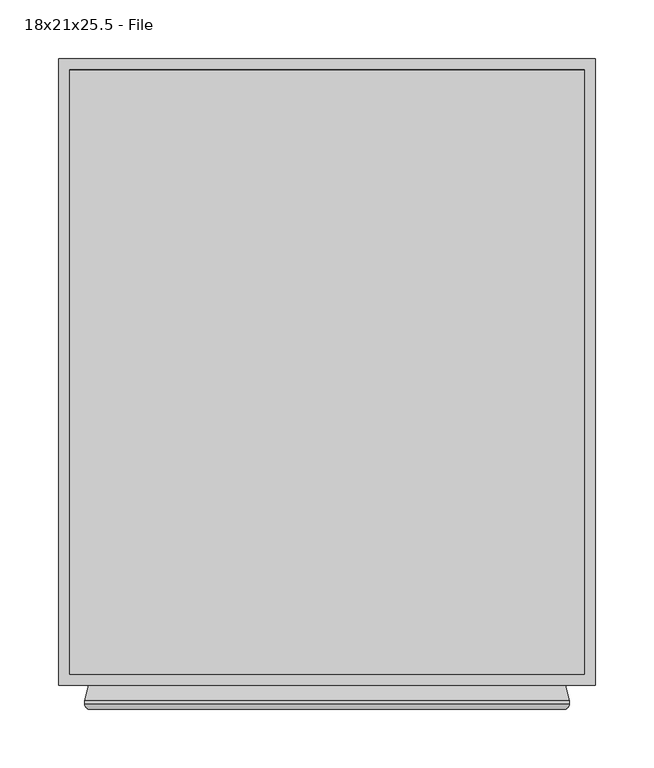
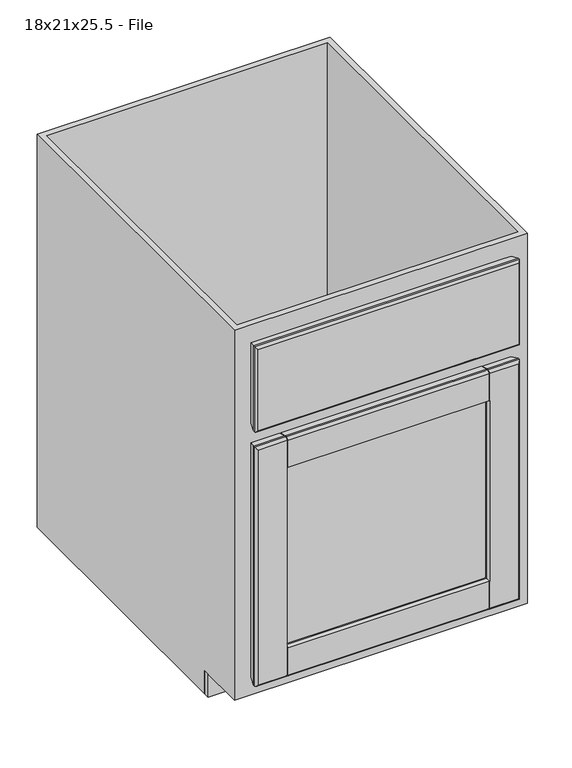
"""IFC4 building model written with IfcOpenShell, lengths in millimetres: furniture geometry, Cabinet-Base-Merillat-Single_Door-Marlin : 18x21x25.5 - File."""

from ifc_helpers import new_model, si_unit, frame, origin, origin_with_axes, place, context, project, spatial, polyline, circle_curve, ellipse_curve, outline, extrude, faceted_brep, source, transform, mapped, element, save
from ifc_brep_helpers import plane_surface, cylinder_surface, advanced_brep


def furniture_18x21x25_5_file_292c1ec0(model_context):
    return source(origin(), model_context, "Body", "SolidModel", [
        advanced_brep(
        [(225.1127049, -625.4496, 457.2), (222.0162124, -629.92, 454.1035075), (222.0162124, -629.92, 66.5964925), (225.1127049, -625.4496, 63.5), (225.1127049, -622.681, 63.5), (225.1127049, -622.681, 457.2), (221.6075049, -609.6, 67.0052), (221.6075049, -609.6, 453.6948), (176.9115422, -609.6, 408.9988372), (176.9115422, -609.6, 111.7011628), (176.5414105, -610.39375, 112.0712945), (174.4602514, -614.85681, 114.1524535), (174.4602514, -614.85681, 406.5475465), (176.5414105, -610.39375, 408.6287055), (175.8600209, -617.0969093, 112.752684), (175.8600209, -617.0969093, 407.947316), (190.1877049, -617.347, 98.425), (190.1877049, -617.347, 422.275), (190.1877049, -622.173, 98.425), (190.1877049, -622.173, 422.275), (175.8600209, -622.4230907, 112.752684), (175.8600209, -622.4230907, 407.947316), (174.4602514, -624.66319, 114.1524535), (174.4602514, -624.66319, 406.5475465), (176.5414105, -629.12625, 112.0712945), (176.9086747, -629.9138508, 111.7040302), (176.9115422, -629.92, 408.9988372), (176.5414105, -629.12625, 408.6287055), (176.9086747, -629.92, 66.5964925), (176.9086747, -625.4496, 63.5), (-184.5408026, -629.92, 66.5964925), (-187.6372951, -625.4496, 63.5), (-139.4730764, -625.4496, 63.5), (-139.4730764, -629.92, 66.5964925), (175.3211747, -625.4496, 63.5), (175.3211747, -629.92, 66.5964925), (-137.8855764, -629.92, 66.5964925), (-137.8855764, -625.4496, 63.5), (176.9086747, -622.681, 63.5), (-187.6372951, -622.681, 63.5), (-139.4730764, -622.681, 63.5), (175.3211747, -622.681, 63.5), (-137.8855764, -622.681, 63.5), (176.9086747, -609.6, 67.0052), (-184.1320951, -609.6, 67.0052), (-139.4730764, -609.6, 67.0052), (175.3211747, -609.6, 67.0052), (-137.8855764, -609.6, 67.0052), (-136.9848416, -614.85681, 114.1524535), (175.3211747, -610.39375, 112.0712945), (175.3211747, -609.6, 111.7011628), (-137.8855764, -609.6, 111.7011628), (-137.8855764, -610.39375, 112.0712945), (-139.0660006, -610.39375, 112.0712945), (-138.384611, -617.0969093, 112.752684), (-152.7122951, -617.347, 98.425), (-152.7122951, -622.173, 98.425), (-138.384611, -622.4230907, 112.752684), (-136.9848416, -624.66319, 114.1524535), (-139.0660006, -629.12625, 112.0712945), (-137.8855764, -629.12625, 112.0712945), (-137.8855764, -629.92, 111.7011628), (175.3211747, -629.92, 111.7011628), (175.3211747, -629.12625, 112.0712945), (-184.5408026, -629.92, 454.1035075), (-187.6372951, -625.4496, 457.2), (-187.6372951, -622.681, 457.2), (-184.1320951, -609.6, 453.6948), (-139.4361323, -609.6, 111.7011628), (-139.4361323, -609.6, 408.9988372), (-139.0660006, -610.39375, 408.6287055), (-136.9848416, -614.85681, 406.5475465), (-138.384611, -617.0969093, 407.947316), (-152.7122951, -617.347, 422.275), (-152.7122951, -622.173, 422.275), (-138.384611, -622.4230907, 407.947316), (-136.9848416, -624.66319, 406.5475465), (-139.0660006, -629.12625, 408.6287055), (-139.4361323, -629.92, 408.9988372), (-139.4361323, -629.92, 111.7011628), (-139.4730764, -629.92, 454.1035075), (-139.4730764, -625.4496, 457.2), (176.9086747, -625.4496, 457.2), (176.9086747, -629.92, 454.1035075), (-137.8855764, -625.4496, 457.2), (-137.8855764, -629.92, 454.1035075), (175.3211747, -629.92, 454.1035075), (175.3211747, -625.4496, 457.2), (-139.4730764, -622.681, 457.2), (176.9086747, -622.681, 457.2), (-137.8855764, -622.681, 457.2), (175.3211747, -622.681, 457.2), (-139.4730764, -609.6, 453.6948), (176.9086747, -609.6, 453.6948), (-137.8855764, -609.6, 453.6948), (175.3211747, -609.6, 453.6948), (-137.8855764, -609.6, 408.9988372), (175.3211747, -609.6, 408.9988372), (-137.8855764, -610.39375, 408.6287055), (175.3211747, -610.39375, 408.6287055), (175.3211747, -629.12625, 408.6287055), (175.3211747, -629.92, 408.9988372), (-137.8855764, -629.92, 408.9988372), (-137.8855764, -629.12625, 408.6287055), (-137.8855764, -610.39375, 453.0857412), (-137.8855764, -622.7855037, 456.40625), (-137.8855764, -625.4496, 456.40625), (-137.8855764, -629.12625, 453.9526052), (-139.4730764, -629.12625, 408.6287055), (-139.4730764, -629.12625, 453.9526052), (-139.4730764, -625.4496, 456.40625), (-139.4730764, -622.7855037, 456.40625), (-139.4730764, -610.39375, 453.0857412), (-139.4730764, -610.39375, 408.6287055), (176.9086747, -610.39375, 408.6287055), (176.9086747, -610.39375, 453.0857412), (176.9086747, -622.7855037, 456.40625), (176.9086747, -625.4496, 456.40625), (176.9086747, -629.12625, 453.9526052), (176.9086747, -629.12625, 408.6287055), (175.3211747, -629.12625, 453.9526052), (175.3211747, -625.4496, 456.40625), (175.3211747, -622.7855037, 456.40625), (175.3211747, -610.39375, 453.0857412), (176.9086747, -629.12625, 112.0712945), (176.9086747, -629.12625, 66.7473948), (176.9086747, -625.4496, 64.29375), (176.9086747, -622.7855037, 64.29375), (176.9086747, -610.39375, 67.6142588), (176.9086747, -610.39375, 112.0712945), (175.3211747, -610.39375, 67.6142588), (175.3211747, -622.7855037, 64.29375), (175.3211747, -625.4496, 64.29375), (175.3211747, -629.12625, 66.7473948), (-137.8855764, -629.12625, 66.7473948), (-137.8855764, -625.4496, 64.29375), (-137.8855764, -622.7855037, 64.29375), (-137.8855764, -610.39375, 67.6142588), (-139.4730764, -629.12625, 112.0712945), (-139.4730764, -610.39375, 112.0712945), (-139.4730764, -610.39375, 67.6142588), (-139.4730764, -622.7855037, 64.29375), (-139.4730764, -625.4496, 64.29375), (-139.4730764, -629.12625, 66.7473948)],
        [
            (0, 1, ellipse_curve(frame((220.3375049, -625.4496, 452.4248), z_axis=(0.7071067811865475, 0.0, -0.7071067811865475), x_axis=(0.7071067811865474, 0.0, 0.7071067811865476)), 6.7531526, 4.7752)),
            (1, 2),
            (2, 3, ellipse_curve(frame((220.3375049, -625.4496, 68.2752), z_axis=(0.7071067811865475, 0.0, 0.7071067811865475), x_axis=(-0.7071067811865474, 0.0, 0.7071067811865476)), 6.7531526, 4.7752)),
            (3, 0),
            (3, 4),
            (4, 5),
            (5, 0),
            (4, 6),
            (6, 7),
            (7, 5),
            (8, 9),
            (9, 10),
            (10, 11),
            (11, 12),
            (12, 13),
            (13, 8),
            (11, 14, ellipse_curve(frame((175.8875049, -615.5223492, 112.7252), z_axis=(0.7071067811865475, 0.0, 0.7071067811865475), x_axis=(-0.7071067811865474, 0.0, 0.7071067811865476)), 2.2271035, 1.5748)),
            (14, 15),
            (15, 12, ellipse_curve(frame((175.8875049, -615.5223492, 407.9748), z_axis=(0.7071067811865475, 0.0, -0.7071067811865475), x_axis=(0.7071067811865474, 0.0, 0.7071067811865476)), 2.2271035, 1.5748)),
            (14, 16),
            (16, 17),
            (17, 15),
            (16, 18),
            (18, 19),
            (19, 17),
            (18, 20),
            (20, 21),
            (21, 19),
            (20, 22, ellipse_curve(frame((175.8875049, -623.9976508, 112.7252), z_axis=(0.7071067811865475, 0.0, 0.7071067811865475), x_axis=(-0.7071067811865474, 0.0, 0.7071067811865476)), 2.2271035, 1.5748)),
            (22, 23),
            (23, 21, ellipse_curve(frame((175.8875049, -623.9976508, 407.9748), z_axis=(0.7071067811865475, 0.0, -0.7071067811865475), x_axis=(0.7071067811865474, 0.0, 0.7071067811865476)), 2.2271035, 1.5748)),
            (22, 24),
            (24, 25),
            (25, 26),
            (26, 27),
            (27, 23),
            (2, 28),
            (28, 29, circle_curve(frame((176.9086747, -625.4496, 68.2752), z_axis=(1.0, 0.0, 0.0), x_axis=(0.0, 1.0, 0.0)), 4.7752)),
            (29, 3),
            (30, 31, ellipse_curve(frame((-182.8620951, -625.4496, 68.2752), z_axis=(0.7071067811865475, 0.0, -0.7071067811865475), x_axis=(0.7071067811865476, 0.0, 0.7071067811865474)), 6.7531526, 4.7752)),
            (31, 32),
            (32, 33, circle_curve(frame((-139.4730764, -625.4496, 68.2752), z_axis=(-1.0, 0.0, 0.0), x_axis=(0.0, 1.0, 0.0)), 4.7752)),
            (33, 30),
            (34, 35, circle_curve(frame((175.3211747, -625.4496, 68.2752), z_axis=(-1.0, 0.0, 0.0), x_axis=(0.0, 1.0, 0.0)), 4.7752)),
            (35, 36),
            (36, 37, circle_curve(frame((-137.8855764, -625.4496, 68.2752), z_axis=(1.0, 0.0, 0.0), x_axis=(0.0, 1.0, 0.0)), 4.7752)),
            (37, 34),
            (29, 38),
            (38, 4),
            (31, 39),
            (39, 40),
            (40, 32),
            (41, 34),
            (37, 42),
            (42, 41),
            (38, 43),
            (43, 6),
            (39, 44),
            (44, 45),
            (45, 40),
            (46, 41),
            (42, 47),
            (47, 46),
            (48, 11),
            (10, 49),
            (49, 50),
            (50, 51),
            (51, 52),
            (52, 53),
            (53, 48),
            (48, 54, ellipse_curve(frame((-138.4120951, -615.5223492, 112.7252), z_axis=(0.7071067811865475, 0.0, -0.7071067811865475), x_axis=(0.7071067811865476, 0.0, 0.7071067811865474)), 2.2271035, 1.5748)),
            (54, 14),
            (54, 55),
            (55, 16),
            (55, 56),
            (56, 18),
            (56, 57),
            (57, 20),
            (57, 58, ellipse_curve(frame((-138.4120951, -623.9976508, 112.7252), z_axis=(0.7071067811865475, 0.0, -0.7071067811865475), x_axis=(0.7071067811865476, 0.0, 0.7071067811865474)), 2.2271035, 1.5748)),
            (58, 22),
            (58, 59),
            (59, 60),
            (60, 61),
            (61, 62),
            (62, 63),
            (63, 24),
            (30, 64),
            (64, 65, ellipse_curve(frame((-182.8620951, -625.4496, 452.4248), z_axis=(-0.7071067811865475, 0.0, -0.7071067811865475), x_axis=(0.7071067811865474, 0.0, -0.7071067811865476)), 6.7531526, 4.7752)),
            (65, 31),
            (65, 66),
            (66, 39),
            (66, 67),
            (67, 44),
            (68, 69),
            (69, 70),
            (70, 71),
            (71, 48),
            (53, 68),
            (71, 72, ellipse_curve(frame((-138.4120951, -615.5223492, 407.9748), z_axis=(-0.7071067811865475, 0.0, -0.7071067811865475), x_axis=(0.7071067811865474, 0.0, -0.7071067811865476)), 2.2271035, 1.5748)),
            (72, 54),
            (72, 73),
            (73, 55),
            (73, 74),
            (74, 56),
            (74, 75),
            (75, 57),
            (75, 76, ellipse_curve(frame((-138.4120951, -623.9976508, 407.9748), z_axis=(-0.7071067811865475, 0.0, -0.7071067811865475), x_axis=(0.7071067811865474, 0.0, -0.7071067811865476)), 2.2271035, 1.5748)),
            (76, 58),
            (76, 77),
            (77, 78),
            (78, 79),
            (79, 59),
            (64, 80),
            (80, 81, circle_curve(frame((-139.4730764, -625.4496, 452.4248), z_axis=(-1.0, 0.0, 0.0), x_axis=(0.0, 1.0, 0.0)), 4.7752)),
            (81, 65),
            (0, 82),
            (82, 83, circle_curve(frame((176.9086747, -625.4496, 452.4248), z_axis=(1.0, 0.0, 0.0), x_axis=(0.0, 1.0, 0.0)), 4.7752)),
            (83, 1),
            (84, 85, circle_curve(frame((-137.8855764, -625.4496, 452.4248), z_axis=(1.0, 0.0, 0.0), x_axis=(0.0, 1.0, 0.0)), 4.7752)),
            (85, 86),
            (86, 87, circle_curve(frame((175.3211747, -625.4496, 452.4248), z_axis=(-1.0, 0.0, 0.0), x_axis=(0.0, 1.0, 0.0)), 4.7752)),
            (87, 84),
            (81, 88),
            (88, 66),
            (5, 89),
            (89, 82),
            (90, 84),
            (87, 91),
            (91, 90),
            (88, 92),
            (92, 67),
            (7, 93),
            (93, 89),
            (94, 90),
            (91, 95),
            (95, 94),
            (43, 9),
            (8, 93),
            (92, 69),
            (68, 45),
            (96, 94),
            (95, 97),
            (97, 96),
            (50, 46),
            (47, 51),
            (12, 71),
            (70, 98),
            (98, 96),
            (97, 99),
            (99, 13),
            (15, 72),
            (17, 73),
            (19, 74),
            (21, 75),
            (23, 76),
            (27, 100),
            (100, 101),
            (101, 102),
            (102, 103),
            (103, 77),
            (83, 26),
            (25, 28),
            (33, 79),
            (78, 80),
            (85, 102),
            (101, 86),
            (35, 62),
            (61, 36),
            (98, 104),
            (104, 105),
            (105, 106),
            (106, 107, circle_curve(frame((-137.8855764, -625.4496, 452.4248), z_axis=(1.0, 0.0, 0.0), x_axis=(0.0, 0.0, 1.0)), 3.98145)),
            (107, 103),
            (78, 108),
            (108, 109),
            (109, 110, circle_curve(frame((-139.4730764, -625.4496, 452.4248), z_axis=(-1.0, 0.0, 0.0), x_axis=(0.0, 0.0, 1.0)), 3.98145)),
            (110, 111),
            (111, 112),
            (112, 113),
            (113, 69),
            (77, 108),
            (107, 109),
            (106, 110),
            (105, 111),
            (104, 112),
            (70, 113),
            (8, 114),
            (114, 115),
            (115, 116),
            (116, 117),
            (117, 118, circle_curve(frame((176.9086747, -625.4496, 452.4248), z_axis=(1.0, 0.0, 0.0), x_axis=(0.0, 0.0, 1.0)), 3.98145)),
            (118, 119),
            (119, 26),
            (100, 120),
            (120, 121, circle_curve(frame((175.3211747, -625.4496, 452.4248), z_axis=(-1.0, 0.0, 0.0), x_axis=(0.0, 0.0, 1.0)), 3.98145)),
            (121, 122),
            (122, 123),
            (123, 99),
            (119, 27),
            (118, 120),
            (117, 121),
            (116, 122),
            (115, 123),
            (114, 13),
            (25, 124),
            (124, 125),
            (125, 126, circle_curve(frame((176.9086747, -625.4496, 68.2752), z_axis=(1.0, 0.0, 0.0), x_axis=(0.0, 0.0, 1.0)), 3.98145)),
            (126, 127),
            (127, 128),
            (128, 129),
            (129, 9),
            (49, 130),
            (130, 131),
            (131, 132),
            (132, 133, circle_curve(frame((175.3211747, -625.4496, 68.2752), z_axis=(-1.0, 0.0, 0.0), x_axis=(0.0, 0.0, 1.0)), 3.98145)),
            (133, 63),
            (129, 10),
            (128, 130),
            (127, 131),
            (126, 132),
            (125, 133),
            (124, 24),
            (60, 134),
            (134, 135, circle_curve(frame((-137.8855764, -625.4496, 68.2752), z_axis=(1.0, 0.0, 0.0), x_axis=(0.0, 0.0, 1.0)), 3.98145)),
            (135, 136),
            (136, 137),
            (137, 52),
            (138, 79),
            (68, 139),
            (139, 140),
            (140, 141),
            (141, 142),
            (142, 143, circle_curve(frame((-139.4730764, -625.4496, 68.2752), z_axis=(-1.0, 0.0, 0.0), x_axis=(0.0, 0.0, 1.0)), 3.98145)),
            (143, 138),
            (138, 59),
            (53, 139),
            (137, 140),
            (136, 141),
            (135, 142),
            (134, 143),
        ],
        [
            cylinder_surface(frame((220.3375049, -625.4496, 457.2), z_axis=(0.0, 0.0, 1.0), x_axis=(0.0, 1.0, 0.0)), 4.7752),
            plane_surface(frame((225.1127049, -625.4496, 457.2), z_axis=(1.0, 0.0, 0.0), x_axis=(0.0, 0.0, -1.0))),
            plane_surface(frame((225.1127049, -622.681, 457.2), z_axis=(0.9659229350723619, 0.25882983502910506, 0.0), x_axis=(0.0, 0.0, -1.0))),
            plane_surface(frame((176.9115422, -609.6, 408.9988372), z_axis=(-0.9063077870366099, 0.4226182617407856, 0.0), x_axis=(0.0, 0.0, -1.0))),
            cylinder_surface(frame((175.8875049, -615.5223492, 457.2), z_axis=(0.0, 0.0, 1.0000000000000002), x_axis=(-0.01745240643729364, -0.9998476951563912, 0.0)), 1.5748),
            plane_surface(frame((175.8600209, -617.0969093, 407.947316), z_axis=(-0.017452406437322144, -0.9998476951563906, 0.0), x_axis=(0.0, 0.0, -1.0))),
            plane_surface(frame((190.1877049, -617.347, 422.275), z_axis=(-1.0, 0.0, 0.0), x_axis=(0.0, 0.0, -1.0))),
            plane_surface(frame((190.1877049, -622.173, 422.275), z_axis=(-0.01745240643727848, 0.9998476951563914, 0.0), x_axis=(0.0, 0.0, -1.0))),
            cylinder_surface(frame((175.8875049, -623.9976508, 457.2), z_axis=(0.0, 0.0, 1.0000000000000002), x_axis=(-0.9063077870367326, -0.42261826174052236, 0.0)), 1.5748),
            plane_surface(frame((174.4602514, -624.66319, 406.5475465), z_axis=(-0.9063077870366333, -0.4226182617407352, 0.0), x_axis=(0.0, 0.0, -1.0))),
            cylinder_surface(frame((225.1127049, -625.4496, 68.2752), z_axis=(1.0, 0.0, 0.0), x_axis=(0.0, 1.0, 0.0)), 4.7752),
            plane_surface(frame((225.1127049, -625.4496, 63.5), z_axis=(0.0, 0.0, -1.0), x_axis=(-1.0, 0.0, 0.0))),
            plane_surface(frame((225.1127049, -622.681, 63.5), z_axis=(0.0, 0.25882983502910506, -0.9659229350723619), x_axis=(-1.0, 0.0, 0.0))),
            plane_surface(frame((176.9115422, -609.6, 111.7011628), z_axis=(0.0, 0.4226182617407856, 0.9063077870366099), x_axis=(-1.0, 0.0, 0.0))),
            cylinder_surface(frame((225.1127049, -615.5223492, 112.7252), z_axis=(1.0000000000000002, 0.0, 0.0), x_axis=(0.0, -0.9998476951563912, 0.01745240643729364)), 1.5748),
            plane_surface(frame((175.8600209, -617.0969093, 112.752684), z_axis=(0.0, -0.9998476951563906, 0.017452406437322144), x_axis=(-1.0, 0.0, 0.0))),
            plane_surface(frame((190.1877049, -617.347, 98.425), z_axis=(0.0, 0.0, 1.0), x_axis=(-1.0, 0.0, 0.0))),
            plane_surface(frame((190.1877049, -622.173, 98.425), z_axis=(0.0, 0.9998476951563914, 0.01745240643727848), x_axis=(-1.0, 0.0, 0.0))),
            cylinder_surface(frame((225.1127049, -623.9976508, 112.7252), z_axis=(1.0000000000000002, 0.0, 0.0), x_axis=(0.0, -0.42261826174052236, 0.9063077870367326)), 1.5748),
            plane_surface(frame((174.4602514, -624.66319, 114.1524535), z_axis=(0.0, -0.4226182617407352, 0.9063077870366333), x_axis=(-1.0, 0.0, 0.0))),
            cylinder_surface(frame((-182.8620951, -625.4496, 63.5), z_axis=(0.0, 0.0, -1.0), x_axis=(0.0, 1.0, 0.0)), 4.7752),
            plane_surface(frame((-187.6372951, -625.4496, 63.5), z_axis=(-1.0, 0.0, 0.0), x_axis=(0.0, 0.0, 1.0))),
            plane_surface(frame((-187.6372951, -622.681, 63.5), z_axis=(-0.9659229350723619, 0.25882983502910506, 0.0), x_axis=(0.0, 0.0, 1.0))),
            plane_surface(frame((-139.4361323, -609.6, 111.7011628), z_axis=(0.9063077870366099, 0.4226182617407856, 0.0), x_axis=(0.0, 0.0, 1.0))),
            cylinder_surface(frame((-138.4120951, -615.5223492, 63.5), z_axis=(0.0, 0.0, -1.0000000000000002), x_axis=(0.01745240643729364, -0.9998476951563912, 0.0)), 1.5748),
            plane_surface(frame((-138.384611, -617.0969093, 112.752684), z_axis=(0.017452406437322144, -0.9998476951563906, 0.0), x_axis=(0.0, 0.0, 1.0))),
            plane_surface(frame((-152.7122951, -617.347, 98.425), z_axis=(1.0, 0.0, 0.0), x_axis=(0.0, 0.0, 1.0))),
            plane_surface(frame((-152.7122951, -622.173, 98.425), z_axis=(0.01745240643727848, 0.9998476951563914, 0.0), x_axis=(0.0, 0.0, 1.0))),
            cylinder_surface(frame((-138.4120951, -623.9976508, 63.5), z_axis=(0.0, 0.0, -1.0000000000000002), x_axis=(0.9063077870367326, -0.42261826174052236, 0.0)), 1.5748),
            plane_surface(frame((-136.9848416, -624.66319, 114.1524535), z_axis=(0.9063077870366333, -0.4226182617407352, 0.0), x_axis=(0.0, 0.0, 1.0))),
            cylinder_surface(frame((-187.6372951, -625.4496, 452.4248), z_axis=(-1.0, 0.0, 0.0), x_axis=(0.0, 1.0, 0.0)), 4.7752),
            plane_surface(frame((-187.6372951, -625.4496, 457.2), z_axis=(0.0, 0.0, 1.0), x_axis=(1.0, 0.0, 0.0))),
            plane_surface(frame((-187.6372951, -622.681, 457.2), z_axis=(0.0, 0.25882983502910506, 0.9659229350723619), x_axis=(1.0, 0.0, 0.0))),
            plane_surface(frame((-184.1320951, -609.6, 453.6948), z_axis=(0.0, 1.0, 0.0), x_axis=(1.0, 0.0, 0.0))),
            plane_surface(frame((-139.4361323, -609.6, 408.9988372), z_axis=(0.0, 0.4226182617407856, -0.9063077870366099), x_axis=(1.0, 0.0, 0.0))),
            cylinder_surface(frame((-187.6372951, -615.5223492, 407.9748), z_axis=(-1.0000000000000002, 0.0, 0.0), x_axis=(0.0, -0.9998476951563912, -0.01745240643729364)), 1.5748),
            plane_surface(frame((-138.384611, -617.0969093, 407.947316), z_axis=(0.0, -0.9998476951563906, -0.017452406437322144), x_axis=(1.0, 0.0, 0.0))),
            plane_surface(frame((-152.7122951, -617.347, 422.275), z_axis=(0.0, 0.0, -1.0), x_axis=(1.0, 0.0, 0.0))),
            plane_surface(frame((-152.7122951, -622.173, 422.275), z_axis=(0.0, 0.9998476951563914, -0.01745240643727848), x_axis=(1.0, 0.0, 0.0))),
            cylinder_surface(frame((-187.6372951, -623.9976508, 407.9748), z_axis=(-1.0000000000000002, 0.0, 0.0), x_axis=(0.0, -0.42261826174052236, -0.9063077870367326)), 1.5748),
            plane_surface(frame((-136.9848416, -624.66319, 406.5475465), z_axis=(0.0, -0.4226182617407352, -0.9063077870366333), x_axis=(1.0, 0.0, 0.0))),
            plane_surface(frame((-139.4361323, -629.92, 408.9988372), z_axis=(0.0, -1.0, 0.0), x_axis=(1.0, 0.0, 0.0))),
            plane_surface(frame((-137.8855764, -629.92, 408.9988372), z_axis=(-1.0000000000000002, 0.0, 0.0), x_axis=(0.0, 0.9063077870366303, -0.4226182617407418))),
            plane_surface(frame((-139.4730764, -629.92, 408.9988372), z_axis=(1.0000000000000002, 0.0, 0.0), x_axis=(0.0, -0.9063077870366303, 0.4226182617407418))),
            plane_surface(frame((-137.8855764, -629.92, 408.9988372), z_axis=(0.0, 0.4226182617407418, 0.9063077870366303), x_axis=(-1.0, 0.0, 0.0))),
            plane_surface(frame((-137.8855764, -629.12625, 408.6287055), z_axis=(0.0, -1.0, 0.0), x_axis=(-1.0, 0.0, 0.0))),
            cylinder_surface(frame((-139.4730764, -625.4496, 452.4248), z_axis=(-1.0, 0.0, 0.0), x_axis=(0.0, 0.0, 1.0)), 3.98145),
            plane_surface(frame((-137.8855764, -625.4496, 456.40625), z_axis=(0.0, 0.0, 1.0), x_axis=(-1.0, 0.0, 0.0))),
            plane_surface(frame((-137.8855764, -622.7855037, 456.40625), z_axis=(0.0, 0.25882983502916795, 0.9659229350723451), x_axis=(-1.0, 0.0, 0.0))),
            plane_surface(frame((-137.8855764, -610.39375, 453.0857412), z_axis=(0.0, 1.0, 0.0), x_axis=(-1.0, 0.0, 0.0))),
            plane_surface(frame((-137.8855764, -610.39375, 408.6287055), z_axis=(0.0, -0.4226182617407951, 0.9063077870366054), x_axis=(-1.0, 0.0, 0.0))),
            plane_surface(frame((176.9086747, -629.92, 408.9988372), z_axis=(-1.0, 0.0, 0.0), x_axis=(0.0, 0.9063077870366284, -0.42261826174074574))),
            plane_surface(frame((175.3211747, -629.92, 408.9988372), z_axis=(1.0, 0.0, 0.0), x_axis=(0.0, -0.9063077870366284, 0.42261826174074574))),
            plane_surface(frame((176.9086747, -629.92, 408.9988372), z_axis=(0.0, 0.42261826174074574, 0.9063077870366284), x_axis=(-1.0, 0.0, 0.0))),
            plane_surface(frame((176.9086747, -629.12625, 408.6287055), z_axis=(0.0, -1.0, 0.0), x_axis=(-1.0, 0.0, 0.0))),
            cylinder_surface(frame((175.3211747, -625.4496, 452.4248), z_axis=(-1.0, 0.0, 0.0), x_axis=(0.0, 0.0, 1.0)), 3.98145),
            plane_surface(frame((176.9086747, -625.4496, 456.40625), z_axis=(0.0, 0.0, 1.0), x_axis=(-1.0, 0.0, 0.0))),
            plane_surface(frame((176.9086747, -622.7855037, 456.40625), z_axis=(0.0, 0.25882983502917023, 0.9659229350723445), x_axis=(-1.0, 0.0, 0.0))),
            plane_surface(frame((176.9086747, -610.39375, 453.0857412), z_axis=(0.0, 1.0, 0.0), x_axis=(-1.0, 0.0, 0.0))),
            plane_surface(frame((176.9086747, -610.39375, 408.6287055), z_axis=(0.0, -0.4226182617408056, 0.9063077870366005), x_axis=(-1.0, 0.0, 0.0))),
            plane_surface(frame((176.9086747, -625.4496, 73.0504), z_axis=(-1.0, 0.0, 0.0), x_axis=(0.0, -1.0, 0.0))),
            plane_surface(frame((175.3211747, -625.4496, 73.0504), z_axis=(1.0, 0.0, 0.0), x_axis=(0.0, 1.0, 0.0))),
            plane_surface(frame((176.9086747, -609.6, 111.7011628), z_axis=(0.0, -0.4226182617407918, -0.906307787036607), x_axis=(-1.0, 0.0, 0.0))),
            plane_surface(frame((176.9086747, -610.39375, 112.0712945), z_axis=(0.0, 1.0, 0.0), x_axis=(-1.0, 0.0, 0.0))),
            plane_surface(frame((176.9086747, -610.39375, 67.6142588), z_axis=(0.0, 0.25882983502943885, -0.9659229350722724), x_axis=(-1.0, 0.0, 0.0))),
            plane_surface(frame((176.9086747, -622.7855037, 64.29375), z_axis=(0.0, 0.0, -1.0), x_axis=(-1.0, 0.0, 0.0))),
            cylinder_surface(frame((175.3211747, -625.4496, 68.2752), z_axis=(-1.0, 0.0, 0.0), x_axis=(0.0, 0.0, 1.0)), 3.98145),
            plane_surface(frame((176.9086747, -629.12625, 66.7473948), z_axis=(0.0, -1.0, 0.0), x_axis=(-1.0, 0.0, 0.0))),
            plane_surface(frame((176.9086747, -629.12625, 112.0712945), z_axis=(0.0, 0.42261826174073464, -0.9063077870366336), x_axis=(-1.0, 0.0, 0.0))),
            plane_surface(frame((-137.8855764, -629.12625, 112.0712945), z_axis=(-1.0, 0.0, 0.0), x_axis=(0.0, -0.9063077870366311, -0.4226182617407399))),
            plane_surface(frame((-139.4730764, -629.12625, 112.0712945), z_axis=(1.0, 0.0, 0.0), x_axis=(0.0, 0.9063077870366311, 0.4226182617407399))),
            plane_surface(frame((-137.8855764, -629.12625, 112.0712945), z_axis=(0.0, 0.4226182617407399, -0.9063077870366311), x_axis=(-1.0, 0.0, 0.0))),
            plane_surface(frame((-137.8855764, -609.6, 111.7011628), z_axis=(0.0, -0.42261826174079353, -0.9063077870366061), x_axis=(-1.0, 0.0, 0.0))),
            plane_surface(frame((-137.8855764, -610.39375, 112.0712945), z_axis=(0.0, 1.0, 0.0), x_axis=(-1.0, 0.0, 0.0))),
            plane_surface(frame((-137.8855764, -610.39375, 67.6142588), z_axis=(0.0, 0.2588298350294384, -0.9659229350722726), x_axis=(-1.0, 0.0, 0.0))),
            plane_surface(frame((-137.8855764, -622.7855037, 64.29375), z_axis=(0.0, 0.0, -1.0), x_axis=(-1.0, 0.0, 0.0))),
            cylinder_surface(frame((-139.4730764, -625.4496, 68.2752), z_axis=(-1.0, 0.0, 0.0), x_axis=(0.0, 0.0, 1.0)), 3.98145),
            plane_surface(frame((-137.8855764, -629.12625, 66.7473948), z_axis=(0.0, -1.0, 0.0), x_axis=(-1.0, 0.0, 0.0))),
        ],
        [
            (0, [[1, 2, 3, 4]]),
            (1, [[-4, 5, 6, 7]]),
            (2, [[-6, 8, 9, 10]]),
            (3, [[11, 12, 13, 14, 15, 16]]),
            (4, [[-14, 17, 18, 19]]),
            (5, [[-18, 20, 21, 22]]),
            (6, [[-21, 23, 24, 25]]),
            (7, [[-24, 26, 27, 28]]),
            (8, [[-27, 29, 30, 31]]),
            (9, [[-30, 32, 33, 34, 35, 36]]),
            (10, [[-3, 37, 38, 39]]),
            (10, [[40, 41, 42, 43]]),
            (10, [[44, 45, 46, 47]]),
            (11, [[-5, -39, 48, 49]]),
            (11, [[50, 51, 52, -41]]),
            (11, [[53, -47, 54, 55]]),
            (12, [[-8, -49, 56, 57]]),
            (12, [[58, 59, 60, -51]]),
            (12, [[61, -55, 62, 63]]),
            (13, [[64, -13, 65, 66, 67, 68, 69, 70]]),
            (14, [[-17, -64, 71, 72]]),
            (15, [[-20, -72, 73, 74]]),
            (16, [[-23, -74, 75, 76]]),
            (17, [[-26, -76, 77, 78]]),
            (18, [[-29, -78, 79, 80]]),
            (19, [[-80, 81, 82, 83, 84, 85, 86, -32]]),
            (20, [[-40, 87, 88, 89]]),
            (21, [[-50, -89, 90, 91]]),
            (22, [[-58, -91, 92, 93]]),
            (23, [[94, 95, 96, 97, -70, 98]]),
            (24, [[-71, -97, 99, 100]]),
            (25, [[-73, -100, 101, 102]]),
            (26, [[-75, -102, 103, 104]]),
            (27, [[-77, -104, 105, 106]]),
            (28, [[-79, -106, 107, 108]]),
            (29, [[-108, 109, 110, 111, 112, -81]]),
            (30, [[-88, 113, 114, 115]]),
            (30, [[-1, 116, 117, 118]]),
            (30, [[119, 120, 121, 122]]),
            (31, [[-90, -115, 123, 124]]),
            (31, [[-7, 125, 126, -116]]),
            (31, [[127, -122, 128, 129]]),
            (32, [[-92, -124, 130, 131]]),
            (32, [[-10, 132, 133, -125]]),
            (32, [[134, -129, 135, 136]]),
            (33, [[-9, -57, 137, -11, 138, -132]]),
            (33, [[-93, -131, 139, -94, 140, -59]]),
            (33, [[141, -136, 142, 143]]),
            (33, [[144, -63, 145, -67]]),
            (34, [[146, -96, 147, 148, -143, 149, 150, -15]]),
            (35, [[-19, 151, -99, -146]]),
            (36, [[-22, 152, -101, -151]]),
            (37, [[-25, 153, -103, -152]]),
            (38, [[-28, 154, -105, -153]]),
            (39, [[-31, 155, -107, -154]]),
            (40, [[-155, -36, 156, 157, 158, 159, 160, -109]]),
            (41, [[-2, -118, 161, -34, 162, -37]]),
            (41, [[-87, -43, 163, -111, 164, -113]]),
            (41, [[165, -158, 166, -120]]),
            (41, [[167, -84, 168, -45]]),
            (42, [[169, 170, 171, 172, 173, -159, -165, -119, -127, -134, -141, -148]]),
            (43, [[174, 175, 176, 177, 178, 179, 180, -139, -130, -123, -114, -164]]),
            (44, [[-174, -110, 181]]),
            (45, [[-173, 182, -175, -181, -160]]),
            (46, [[-172, 183, -176, -182]]),
            (47, [[-171, 184, -177, -183]]),
            (48, [[-170, 185, -178, -184]]),
            (49, [[-169, -147, 186, -179, -185]]),
            (50, [[-180, -186, -95]]),
            (51, [[187, 188, 189, 190, 191, 192, 193, -161, -117, -126, -133, -138]]),
            (52, [[194, 195, 196, 197, 198, -149, -142, -135, -128, -121, -166, -157]]),
            (53, [[-193, 199, -35]]),
            (54, [[-192, 200, -194, -156, -199]]),
            (55, [[-191, 201, -195, -200]]),
            (56, [[-190, 202, -196, -201]]),
            (57, [[-189, 203, -197, -202]]),
            (58, [[-188, 204, -150, -198, -203]]),
            (59, [[-187, -16, -204]]),
            (60, [[205, 206, 207, 208, 209, 210, 211, -137, -56, -48, -38, -162]]),
            (61, [[212, 213, 214, 215, 216, -85, -167, -44, -53, -61, -144, -66]]),
            (62, [[-211, 217, -12]]),
            (63, [[-210, 218, -212, -65, -217]]),
            (64, [[-209, 219, -213, -218]]),
            (65, [[-208, 220, -214, -219]]),
            (66, [[-207, 221, -215, -220]]),
            (67, [[-206, 222, -86, -216, -221]]),
            (68, [[-205, -33, -222]]),
            (69, [[223, 224, 225, 226, 227, -68, -145, -62, -54, -46, -168, -83]]),
            (70, [[228, -163, -42, -52, -60, -140, 229, 230, 231, 232, 233, 234]]),
            (71, [[-228, 235, -112]]),
            (72, [[-229, -98, 236]]),
            (73, [[-227, 237, -230, -236, -69]]),
            (74, [[-226, 238, -231, -237]]),
            (75, [[-225, 239, -232, -238]]),
            (76, [[-224, 240, -233, -239]]),
            (77, [[-223, -82, -235, -234, -240]]),
        ],
    ),
        extrude(outline(polyline([(-152.7122951, -622.173), (-152.7122951, -617.347), (190.1877049, -617.347), (190.1877049, -622.173), (-152.7122951, -622.173)])), frame((0.0, 0.0, 98.425), z_axis=(0.0, 0.0, 1.0), x_axis=(1.0, 0.0, 0.0)), (0.0, 0.0, 1.0), 323.85),
        advanced_brep(
        [(-184.5408026, -629.92, 619.2035075), (-184.5408026, -629.92, 485.6964925), (222.0162124, -629.92, 485.6964925), (222.0162124, -629.92, 619.2035075), (-184.1320951, -609.6, 486.1052), (-184.1320951, -609.6, 618.7948), (221.6075049, -609.6, 618.7948), (221.6075049, -609.6, 486.1052), (-187.6372951, -625.4496, 622.3), (-187.6372951, -622.681, 622.3), (-187.6372951, -622.681, 482.6), (-187.6372951, -625.4496, 482.6), (225.1127049, -622.681, 482.6), (225.1127049, -625.4496, 482.6), (225.1127049, -622.681, 622.3), (225.1127049, -625.4496, 622.3)],
        [
            (0, 1),
            (1, 2),
            (2, 3),
            (3, 0),
            (4, 5),
            (5, 6),
            (6, 7),
            (7, 4),
            (8, 9),
            (9, 10),
            (10, 11),
            (11, 8),
            (10, 12),
            (12, 13),
            (13, 11),
            (12, 14),
            (14, 15),
            (15, 13),
            (8, 15),
            (14, 9),
            (11, 1, ellipse_curve(frame((-182.8620951, -625.4496, 487.3752), z_axis=(-0.7071067811865475, 0.0, 0.7071067811865475), x_axis=(-0.7071067811865474, 0.0, -0.7071067811865476)), 6.7531526, 4.7752)),
            (0, 8, ellipse_curve(frame((-182.8620951, -625.4496, 617.5248), z_axis=(-0.7071067811865475, 0.0, -0.7071067811865475), x_axis=(0.7071067811865474, 0.0, -0.7071067811865476)), 6.7531526, 4.7752)),
            (4, 10),
            (9, 5),
            (13, 2, ellipse_curve(frame((220.3375049, -625.4496, 487.3752), z_axis=(-0.7071067811865475, 0.0, -0.7071067811865475), x_axis=(0.7071067811865476, 0.0, -0.7071067811865474)), 6.7531526, 4.7752)),
            (7, 12),
            (15, 3, ellipse_curve(frame((220.3375049, -625.4496, 617.5248), z_axis=(0.7071067811865475, 0.0, -0.7071067811865475), x_axis=(0.7071067811865474, 0.0, 0.7071067811865476)), 6.7531526, 4.7752)),
            (6, 14),
        ],
        [
            plane_surface(frame((-187.6372951, -629.92, 622.3), z_axis=(0.0, -1.0, 0.0), x_axis=(0.0, 0.0, -1.0))),
            plane_surface(frame((-187.6372951, -609.6, 622.3), z_axis=(0.0, 1.0, 0.0), x_axis=(0.0, 0.0, 1.0))),
            plane_surface(frame((-187.6372951, -629.92, 622.3), z_axis=(-1.0, 0.0, 0.0), x_axis=(0.0, 1.0, 0.0))),
            plane_surface(frame((-187.6372951, -629.92, 482.6), z_axis=(0.0, 0.0, -1.0), x_axis=(0.0, 1.0, 0.0))),
            plane_surface(frame((225.1127049, -629.92, 482.6), z_axis=(1.0, 0.0, 0.0), x_axis=(0.0, 1.0, 0.0))),
            plane_surface(frame((225.1127049, -629.92, 622.3), z_axis=(0.0, 0.0, 1.0), x_axis=(0.0, 1.0, 0.0))),
            cylinder_surface(frame((-182.8620951, -625.4496, 622.3), z_axis=(0.0, 0.0, -1.0), x_axis=(0.0, 1.0, 0.0)), 4.7752),
            plane_surface(frame((-187.6372951, -622.681, 622.3), z_axis=(-0.9659229350723619, 0.25882983502910506, 0.0), x_axis=(0.0, 0.0, -1.0))),
            cylinder_surface(frame((-187.6372951, -625.4496, 487.3752), z_axis=(1.0, 0.0, 0.0), x_axis=(0.0, 1.0, 0.0)), 4.7752),
            plane_surface(frame((-187.6372951, -622.681, 482.6), z_axis=(0.0, 0.25882983502910506, -0.9659229350723619), x_axis=(1.0, 0.0, 0.0))),
            cylinder_surface(frame((220.3375049, -625.4496, 482.6), z_axis=(0.0, 0.0, 1.0), x_axis=(0.0, 1.0, 0.0)), 4.7752),
            plane_surface(frame((225.1127049, -622.681, 482.6), z_axis=(0.9659229350723619, 0.25882983502910506, 0.0), x_axis=(0.0, 0.0, 1.0))),
            cylinder_surface(frame((225.1127049, -625.4496, 617.5248), z_axis=(-1.0, 0.0, 0.0), x_axis=(0.0, 1.0, 0.0)), 4.7752),
            plane_surface(frame((225.1127049, -622.681, 622.3), z_axis=(0.0, 0.25882983502910506, 0.9659229350723619), x_axis=(-1.0, 0.0, 0.0))),
        ],
        [
            (0, [[1, 2, 3, 4]]),
            (1, [[5, 6, 7, 8]]),
            (2, [[9, 10, 11, 12]]),
            (3, [[-11, 13, 14, 15]]),
            (4, [[-14, 16, 17, 18]]),
            (5, [[-9, 19, -17, 20]]),
            (6, [[21, -1, 22, -12]]),
            (7, [[23, -10, 24, -5]]),
            (8, [[-21, -15, 25, -2]]),
            (9, [[-23, -8, 26, -13]]),
            (10, [[-25, -18, 27, -3]]),
            (11, [[-26, -7, 28, -16]]),
            (12, [[-22, -4, -27, -19]]),
            (13, [[-24, -20, -28, -6]]),
        ],
    ),
        extrude(outline(polyline([(-209.8622951, -538.95625), (-209.8622951, -529.43125), (247.3377049, -529.43125), (247.3377049, -538.95625), (-209.8622951, -538.95625)])), origin_with_axes(), (0.0, 0.0, 1.0), 38.1),
        faceted_brep([(247.3377049, -76.2, 0.0), (247.3377049, -529.43125, 0.0), (237.8127049, -529.43125, 0.0), (237.8127049, -85.725, 0.0), (-200.3372951, -85.725, 0.0), (-200.3372951, -529.43125, 0.0), (-209.8622951, -529.43125, 0.0), (-209.8622951, -76.2, 0.0), (-209.8622951, -76.2, 647.7), (247.3377049, -76.2, 647.7), (-209.8622951, -529.43125, 38.1), (-209.8622951, -609.6, 38.1), (-209.8622951, -609.6, 647.7), (247.3377049, -609.6, 647.7), (247.3377049, -609.6, 38.1), (247.3377049, -529.43125, 38.1), (237.8127049, -529.43125, 38.1), (237.8127049, -85.725, 38.1), (237.8127049, -600.075, 647.7), (237.8127049, -85.725, 647.7), (237.8127049, -85.725, 42.8625), (237.8127049, -600.075, 42.8625), (-200.3372951, -529.43125, 38.1), (-200.3372951, -85.725, 38.1), (-200.3372951, -85.725, 647.7), (-200.3372951, -600.075, 647.7), (-200.3372951, -600.075, 42.8625), (-200.3372951, -85.725, 42.8625)], [[[0, 1, 2, 3, 4, 5, 6, 7]], [[0, 7, 8, 9]], [[7, 6, 10, 11, 12, 8]], [[1, 0, 9, 13, 14, 15]], [[3, 2, 16, 17]], [[18, 19, 20, 21]], [[6, 5, 22, 10]], [[5, 4, 23, 22]], [[24, 25, 26, 27]], [[4, 3, 17, 23]], [[19, 24, 27, 20]], [[9, 8, 12, 13], [19, 18, 25, 24]], [[14, 11, 10, 22, 23, 17, 16, 15]], [[13, 12, 11, 14]], [[25, 18, 21, 26]], [[21, 20, 27, 26]], [[2, 1, 15, 16]]]),
    ])


if __name__ == "__main__":
    model = new_model("IFC4")
    model_context = context("Model", 3, world=origin())
    ifc_project = project(units=[si_unit("LENGTHUNIT", "METRE", prefix="MILLI")], contexts=[model_context])
    site = spatial("IfcSite", under=ifc_project)
    building = spatial("IfcBuilding", under=site)
    placement = place(None, origin())
    furniture_18x21x25_5_file_shape = furniture_18x21x25_5_file_292c1ec0(model_context)
    element("IfcFurniture", 1, ObjectType="Cabinet-Base-Merillat-Single_Door-Marlin : 18x21x25.5 - File", at=placement, inside=building, context=model_context, shape_type="MappedRepresentation", body=[
        mapped(furniture_18x21x25_5_file_shape, transform((0.0, 0.0, 0.0), x_axis=(1.0, 0.0, 0.0), y_axis=(0.0, 1.0, 0.0), z_axis=(0.0, 0.0, 1.0))),
    ])
    save(model, "model.ifc")

# Revit data of these elements
# Type "Cabinet-Base-Merillat-Single_Door-Marlin : 18x21x25.5 - File"
#   URL = "http://www.merillat.com"
#   Toe Kick Note = "Toe Kick Covering is not included. To be purchased Separately."
#   Product Page URL = "http://www.merillat.com//our-products/rooms/kitchen/"
#   Product Line = "Express"
#   Product Group = "Base Cabinet"
#   Product Documentation Link = "http://merillatbusiness.com/customer-resources/product-line-resources/merillat-classic/"
#   Model = "BWBT18"
#   Manufacturer = "Merillat"
#   Finish = "Wood"
#   Description = "Base Wastebasket Top Mount"
#   Construction Type = "Sink Base Single Door"
#   Cabinet Construction Note = "BWBT18 has two 35 qt. white pastic baskets (no garbage bag tray storage), Door is attached  to wastebasket assembly and is pulled open to access basket"
#   Assembly Code = "C1030410"
#   Top and Bottom Spacing = 0' - 1"
#   Toe Kick Height = 0' - 1 1/2"
#   Toe Kick Depth = 0' - 2 25/32"
#   Depth = 1' - 9"
#   Height = 2' - 1 1/2"
#   Width = 1' - 6"
#   Cabinet Shell = 0' - 0 3/8"
#   Cabinet Drawer Width = 1' - 4 1/4"
#   Cabinet Drawer Height = 0' - 5 1/2"
#   Cabinet Door Width = 1' - 4 1/4"
#   Cabinet Door Height = 1' - 3 1/2"
#   COBie.Type = no
#   Partial Overlay = yes
#   Full Overlay = no
#   Elevation Swing Line = yes
#   Toe Kick Material = Wood - Merillat - Raw Particle Board
#   Door Drawer Material = Wood - Merillat - Pecan(1)
#   Cabinet Material = Wood - Merillat - Pecan(1)
#   Cabinet Drawer Style = element 785883
#   Cabinet Door Style = element 785884
# Element 1 (IfcFurniture, "Cabinet-Base-Merillat-Single_Door-Marlin : 18x21x25.5 - File")
#   Materials on its faces: "Wood - Merillat - Pecan(1)", "Wood - Merillat - Raw Particle Board"
# Materials
#   "Wood - Merillat - Raw Particle Board": class "Plastic", colour RGB 80 80 80, transparency 0, Description = "Plastic Laminate - Navy", Cost = 0
#   "Wood - Merillat - Pecan(1)": class "Wood", colour RGB 108 67 43, transparency 0, Cost = 0
